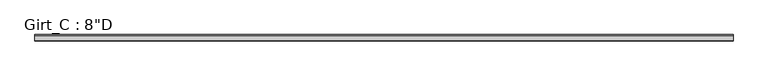
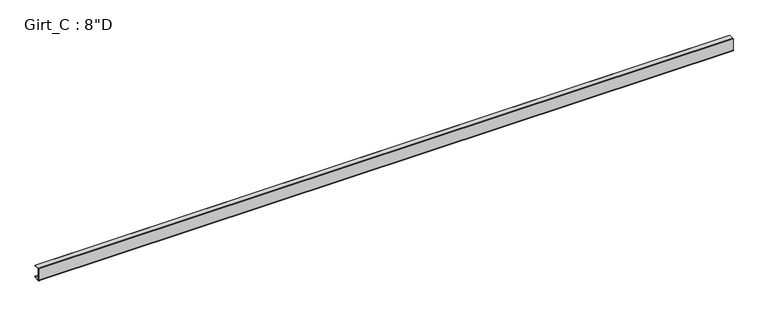
"""IFC4 building model written with IfcOpenShell, lengths in millimetres: beam geometry."""

import ifcopenshell
import ifcopenshell.guid

model = None  # the IFC model being written
_history = None  # IfcOwnerHistory: only IFC2X3 demands one
_inside = {}  # id of a spatial element -> (the spatial element, [elements in it])
_under = {}  # id of a project, library or spatial element -> (it, [spatial elements below it])
_declared = {}  # id of a project -> (the project, [libraries it declares])
_typed = {}  # id of a type object -> (the type object, [elements of that type])
_made_of = {}  # id of a material, layer set ... -> (it, [elements and type objects made of it])


def new_model(schema):
    """Start an empty IFC model of exactly this schema.

    Asked for "IFC4X3", IfcOpenShell would pick the latest addendum, in which some entities
    have other attributes; the version numbers below select the first issue.
    IFC2X3 requires an IfcOwnerHistory on every rooted entity: one is made here for all.
    """
    global model, _history
    if schema == "IFC4X3":
        model = ifcopenshell.file(schema_version=(4, 3, 0, 0))
    else:
        model = ifcopenshell.file(schema=schema)
    _inside.clear()
    _under.clear()
    _declared.clear()
    _typed.clear()
    _made_of.clear()
    _history = None
    if model.schema == "IFC2X3":
        org = make("IfcOrganization", Name="unknown")
        user = make(
            "IfcPersonAndOrganization",
            ThePerson=make("IfcPerson", FamilyName="unknown"),
            TheOrganization=org,
        )
        app = make(
            "IfcApplication",
            ApplicationDeveloper=org,
            Version="unknown",
            ApplicationFullName="unknown",
            ApplicationIdentifier="unknown",
        )
        _history = make(
            "IfcOwnerHistory",
            OwningUser=user,
            OwningApplication=app,
            ChangeAction="ADDED",
            CreationDate=0,
        )
    return model


def make(cls, **values):
    """One entity of the class cls with the attributes given. An attribute that is None is left unset."""
    return model.create_entity(
        cls, **{name: value for name, value in values.items() if value is not None}
    )


def rooted(cls, **values):
    """An entity with a GlobalId (a new one), such as an element, a storey or a relation."""
    return make(cls, GlobalId=ifcopenshell.guid.new(), OwnerHistory=_history, **values)


def si_unit(unit_type, name, prefix=None):
    """IfcSIUnit, for example si_unit("LENGTHUNIT", "METRE", prefix="MILLI")."""
    return make("IfcSIUnit", UnitType=unit_type, Prefix=prefix, Name=name)


def assignment(units):
    """IfcUnitAssignment: the units of a project."""
    return None if units is None else make("IfcUnitAssignment", Units=units)


def point(xyz):
    """IfcCartesianPoint."""
    return None if xyz is None else make("IfcCartesianPoint", Coordinates=xyz)


def direction(xyz):
    """IfcDirection."""
    return None if xyz is None else make("IfcDirection", DirectionRatios=xyz)


def frame(location, z_axis=None, x_axis=None):
    """IfcAxis2Placement3D, a coordinate frame: its origin and axes. An axis left out is left unset."""
    return make(
        "IfcAxis2Placement3D",
        Location=point(location),
        Axis=direction(z_axis),
        RefDirection=direction(x_axis),
    )


def frame_2d(location, x_axis=None):
    """IfcAxis2Placement2D, a coordinate frame in the plane: its origin and x axis."""
    return make(
        "IfcAxis2Placement2D", Location=point(location), RefDirection=direction(x_axis)
    )


def origin():
    """The frame at (0, 0, 0) with its axes left unset."""
    return frame((0.0, 0.0, 0.0))


def place(relative_to, where):
    """IfcLocalPlacement: puts the frame where relative to a parent placement (None: the world)."""
    return make(
        "IfcLocalPlacement", PlacementRelTo=relative_to, RelativePlacement=where
    )


def context(
    kind, dimensions, precision=None, world=None, true_north=None, identifier=None
):
    """IfcGeometricRepresentationContext, for example the 3D "Model" context."""
    return make(
        "IfcGeometricRepresentationContext",
        ContextIdentifier=identifier,
        ContextType=kind,
        CoordinateSpaceDimension=dimensions,
        Precision=precision,
        WorldCoordinateSystem=world,
        TrueNorth=true_north,
    )


def project(units=None, contexts=None):
    """IfcProject with its units and contexts."""
    return rooted(
        "IfcProject",
        Name="project",
        RepresentationContexts=contexts,
        UnitsInContext=assignment(units),
    )


def spatial(cls, under=None, at=None, **own):
    """A site, building, storey or space (cls), placed at a placement, below another one or the project."""
    s = rooted(cls, ObjectPlacement=at, **own)
    if under is not None:
        _under.setdefault(under.id(), (under, []))[1].append(s)
    return s


def polyline(points):
    """IfcPolyline through the points."""
    return make("IfcPolyline", Points=[point(p) for p in points])


def circle_curve(where, radius):
    """IfcCircle in the frame where."""
    return make("IfcCircle", Position=where, Radius=radius)


def trimmed(basis, trim1, trim2, sense, master):
    """IfcTrimmedCurve: the piece of a basis curve between two trims."""
    return make(
        "IfcTrimmedCurve",
        BasisCurve=basis,
        Trim1=trim1,
        Trim2=trim2,
        SenseAgreement=sense,
        MasterRepresentation=master,
    )


def segment(curve, same_sense, transition):
    """IfcCompositeCurveSegment."""
    return make(
        "IfcCompositeCurveSegment",
        Transition=transition,
        SameSense=same_sense,
        ParentCurve=curve,
    )


def composite_curve(segments, self_intersect=None):
    """IfcCompositeCurve: segments joined end to end."""
    return make("IfcCompositeCurve", Segments=segments, SelfIntersect=self_intersect)


def outline(outer, holes=None, kind="AREA"):
    """IfcArbitraryClosedProfileDef: a profile drawn as a closed curve; with holes, ...WithVoids."""
    if holes is None:
        return make("IfcArbitraryClosedProfileDef", ProfileType=kind, OuterCurve=outer)
    return make(
        "IfcArbitraryProfileDefWithVoids",
        ProfileType=kind,
        OuterCurve=outer,
        InnerCurves=holes,
    )


def extrude(swept, where, along, depth):
    """IfcExtrudedAreaSolid: the profile swept, set in the frame where, extruded along a direction by depth."""
    return make(
        "IfcExtrudedAreaSolid",
        SweptArea=swept,
        Position=where,
        ExtrudedDirection=direction(along),
        Depth=depth,
    )


def shape(context_of_items, identifier, shape_type, items):
    """IfcShapeRepresentation: the items that make up one representation, for example the "Body"."""
    return make(
        "IfcShapeRepresentation",
        ContextOfItems=context_of_items,
        RepresentationIdentifier=identifier,
        RepresentationType=shape_type,
        Items=items,
    )


def source(mapping_origin, context_of_items, identifier, shape_type, items):
    """IfcRepresentationMap: a shape defined once, which mapped items show again and again."""
    return make(
        "IfcRepresentationMap",
        MappingOrigin=mapping_origin,
        MappedRepresentation=shape(context_of_items, identifier, shape_type, items),
    )


def transform(
    local_origin,
    x_axis=None,
    y_axis=None,
    z_axis=None,
    scale=None,
    scale2=None,
    scale3=None,
    uniform=True,
):
    """IfcCartesianTransformationOperator3D, or its non-uniform kind. x_axis, y_axis, z_axis: its Axis1, 2, 3."""
    if uniform:
        return make(
            "IfcCartesianTransformationOperator3D",
            Axis1=direction(x_axis),
            Axis2=direction(y_axis),
            LocalOrigin=point(local_origin),
            Scale=scale,
            Axis3=direction(z_axis),
        )
    return make(
        "IfcCartesianTransformationOperator3DnonUniform",
        Axis1=direction(x_axis),
        Axis2=direction(y_axis),
        LocalOrigin=point(local_origin),
        Scale=scale,
        Axis3=direction(z_axis),
        Scale2=scale2,
        Scale3=scale3,
    )


def mapped(mapping_source, mapping_target):
    """IfcMappedItem: shows the shape of a source again, moved by a transform."""
    return make(
        "IfcMappedItem", MappingSource=mapping_source, MappingTarget=mapping_target
    )


def made_of(thing, what):
    """Note that an element or type object is made of a material, layer set ...; save() writes the relation."""
    if what is not None:
        _made_of.setdefault(what.id(), (what, []))[1].append(thing)
    return thing


def element(
    cls,
    number,
    at=None,
    inside=None,
    cuts=None,
    type_object=None,
    material=None,
    context=None,
    identifier="Body",
    shape_type=None,
    held_by="IfcProductDefinitionShape",
    body=None,
    shapes=None,
    **own,
):
    """One element of the class cls, such as IfcWall. Its Tag is "e" and its number.

    at: its placement. inside: the storey or other place that contains it. cuts: it is an
    opening in that element (IfcRelVoidsElement). A single representation is given by context,
    identifier, shape_type and body (its items); several are given by shapes. held_by: the class
    of the entity that holds the representations. save() writes the other relations.
    """
    e = rooted(cls, Tag="e%d" % number, ObjectPlacement=at, **own)
    if body is not None:
        shapes = [shape(context, identifier, shape_type, body)]
    if shapes is not None:
        e.Representation = make(held_by, Representations=shapes)
    if inside is not None:
        _inside.setdefault(inside.id(), (inside, []))[1].append(e)
    if cuts is not None:
        rooted(
            "IfcRelVoidsElement", RelatingBuildingElement=cuts, RelatedOpeningElement=e
        )
    if type_object is not None:
        _typed.setdefault(type_object.id(), (type_object, []))[1].append(e)
    return made_of(e, material)


def aggregate(whole, parts):
    """IfcRelAggregates: a whole, such as a stair, and the parts it consists of."""
    return rooted("IfcRelAggregates", RelatingObject=whole, RelatedObjects=parts)


def save(model, path):
    """Write the relations noted so far, then the file.

    IfcRelAggregates (storeys below a building ...), IfcRelContainedInSpatialStructure (elements
    in a storey), IfcRelDefinesByType, IfcRelAssociatesMaterial and IfcRelDeclares: one each for
    every whole, place, type object, material and project.
    """
    for whole, parts in _under.values():
        aggregate(whole, parts)
    for where, things in _inside.values():
        rooted(
            "IfcRelContainedInSpatialStructure",
            RelatedElements=things,
            RelatingStructure=where,
        )
    for kind, things in _typed.values():
        rooted("IfcRelDefinesByType", RelatedObjects=things, RelatingType=kind)
    for what, things in _made_of.values():
        rooted("IfcRelAssociatesMaterial", RelatedObjects=things, RelatingMaterial=what)
    for by, libraries in _declared.values():
        rooted("IfcRelDeclares", RelatingContext=by, RelatedDefinitions=libraries)
    model.write(path)


def beam_6c181142(model_context):
    return source(origin(), model_context, "Body", "SweptSolid", [
        extrude(outline(composite_curve([segment(polyline([(87.5109375, 101.6), (99.7560415, 87.0068534), (97.6278742, 85.221109), (86.2154765, 98.821875), (3.3005807, 98.821875)]), True, "CONTINUOUS"), segment(trimmed(circle_curve(frame_2d((3.3741066, 96.8381931)), 1.9850441), [point((3.3005807, 98.821875))], [point((1.3890625, 96.8381931))], True, "CARTESIAN"), True, "CONTINUOUS"), segment(polyline([(1.3890625, 96.8381931), (1.3890625, -96.8389339)]), True, "CONTINUOUS"), segment(trimmed(circle_curve(frame_2d((3.3748024, -96.8389339)), 1.9857399), [point((1.3890625, -96.8389339))], [point((3.2694106, -98.821875))], True, "CARTESIAN"), True, "CONTINUOUS"), segment(polyline([(3.2694106, -98.821875), (86.2154765, -98.821875), (97.6510975, -85.1934327), (99.7792647, -86.979177), (87.5109375, -101.6), (3.3734375, -101.6)]), True, "CONTINUOUS"), segment(trimmed(circle_curve(frame_2d((3.3734375, -96.8375)), 4.7625), [point((3.3734375, -101.6))], [point((-1.3890625, -96.8375))], False, "CARTESIAN"), True, "CONTINUOUS"), segment(polyline([(-1.3890625, -96.8375), (-1.3890625, 96.8375)]), True, "CONTINUOUS"), segment(trimmed(circle_curve(frame_2d((3.3734375, 96.8375)), 4.7625), [point((-1.3890625, 96.8375))], [point((3.3734375, 101.6))], False, "CARTESIAN"), True, "CONTINUOUS"), segment(polyline([(3.3734375, 101.6), (87.5109375, 101.6)]), True, "CONTINUOUS")], self_intersect=False)), frame((-5531.374889, 0.0, 0.0), z_axis=(1.0, 0.0, 0.0), x_axis=(0.0, 1.0, 0.0)), (0.0, 0.0, 1.0), 11005.599778),
    ])


if __name__ == "__main__":
    model = new_model("IFC4")
    model_context = context("Model", 3, world=origin())
    ifc_project = project(units=[si_unit("LENGTHUNIT", "METRE", prefix="MILLI")], contexts=[model_context])
    site = spatial("IfcSite", under=ifc_project)
    building = spatial("IfcBuilding", under=site)
    placement = place(None, origin())
    beam_shape = beam_6c181142(model_context)
    element("IfcBeam", 1, ObjectType="Girt_C : 8\"D", at=placement, inside=building, context=model_context, shape_type="MappedRepresentation", body=[
        mapped(beam_shape, transform((0.0, 0.0, 0.0), x_axis=(1.0, 0.0, 0.0), y_axis=(0.0, 1.0, 0.0), z_axis=(0.0, 0.0, 1.0))),
    ])
    save(model, "model.ifc")

# Revit data of these elements
# Type "Girt_C : 8\"D"
#   half leg = 0' - 1 3/4"
#   Web_Thickness = 0' - 0 7/64"
#   Length [instance default] = 10' - 0"
#   Leg_1 = 0' - 3 1/2"
#   Height = 0' - 8"
#   Structural Material [instance default] = none
# Element 1 (IfcBeam, "Girt_C : 8\"D")
#   Structural Material = CEE' SECTION (8.0x3.5C - SEE STRUCT. DWGS)
#   Materials on its faces: "CEE' SECTION (8.0x3.5C - SEE STRUCT. DWGS)"
# Materials
#   "CEE' SECTION (8.0x3.5C - SEE STRUCT. DWGS)": class "Metal", colour RGB 137 146 153, transparency 0, Description = "Steel, mill finish", Cost = 0
